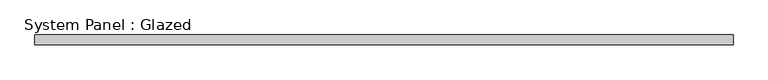
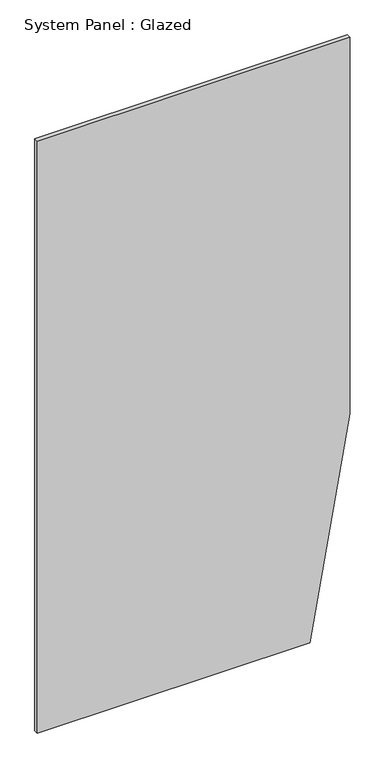
"""IFC4 building model written with IfcOpenShell, lengths in millimetres: plate geometry, System Panel : Glazed."""

from ifc_helpers import new_model, si_unit, frame, origin, place, context, project, spatial, polyline, outline, extrude, source, transform, mapped, element, save


def system_panel_glazed_87679f4c(model_context):
    return source(origin(), model_context, "Body", "SweptSolid", [
        extrude(outline(polyline([(0.0, -914.4), (0.0, 680.3834794), (1332.2432262, 914.4), (3657.6, 914.4), (3657.6, -914.4), (0.0, -914.4)])), frame((0.0, -44.45, 0.0), z_axis=(0.0, 1.0, 0.0), x_axis=(0.0, 0.0, 1.0)), (0.0, 0.0, 1.0), 25.4),
    ])


if __name__ == "__main__":
    model = new_model("IFC4")
    model_context = context("Model", 3, world=origin())
    ifc_project = project(units=[si_unit("LENGTHUNIT", "METRE", prefix="MILLI")], contexts=[model_context])
    site = spatial("IfcSite", under=ifc_project)
    building = spatial("IfcBuilding", under=site)
    placement = place(None, origin())
    system_panel_glazed_shape = system_panel_glazed_87679f4c(model_context)
    element("IfcPlate", 1, ObjectType="System Panel : Glazed", at=placement, inside=building, context=model_context, shape_type="MappedRepresentation", body=[
        mapped(system_panel_glazed_shape, transform((0.0, 0.0, 0.0), x_axis=(1.0, 0.0, 0.0), y_axis=(0.0, 1.0, 0.0), z_axis=(0.0, 0.0, 1.0))),
    ])
    save(model, "model.ifc")

# Revit data of these elements
# Type "System Panel : Glazed"
#   Construction Type Id = "GSP4R"
#   Analytic Construction = "1/8 in Pilkington single glazing"
#   Visual Light Transmittance = 0.9
#   Solar Heat Gain Coefficient = 0.86
#   Heat Transfer Coefficient (U) = 1.18115 BTU/(h·ft²·°F)
#   Define Thermal Properties by = 1
# Element 1 (IfcPlate, "System Panel : Glazed")
#   Materials on its faces: "Glass"
# Materials
#   "Glass": class "Glass", colour RGB 0 128 192, transparency 0.75, Description = "Soda Lime Glass", Cost = 0
